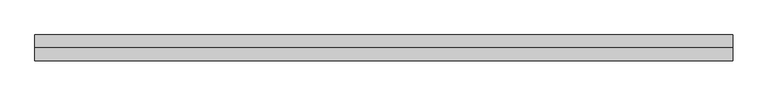
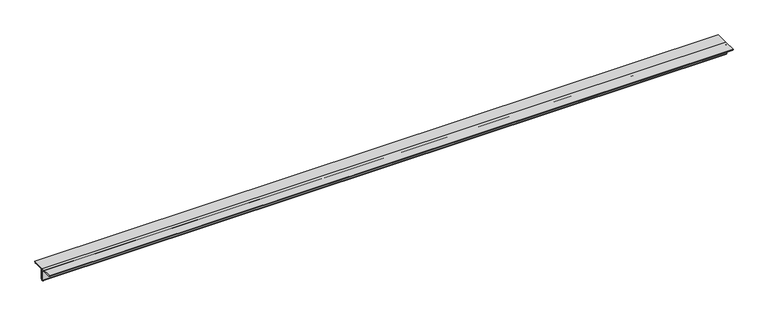
"""IFC4 building model written with IfcOpenShell, lengths in millimetres: member geometry, Steel Framing_2Ls_KS : H_SB_AR_S02_2Ls-100x100x10_VBR1."""

from ifc_helpers import new_model, si_unit, point, frame, frame_2d, origin, place, context, project, spatial, polyline, circle_curve, trimmed, segment, composite_curve, outline, extrude, source, transform, mapped, element, save


def member_a8eb377e(model_context):
    return source(origin(), model_context, "Body", "SweptSolid", [
        extrude(outline(composite_curve([segment(polyline([(0.0, 28.2), (0.0, -71.8)]), True, "CONTINUOUS"), segment(trimmed(circle_curve(frame_2d((0.0, -61.8)), 10.0), [point((0.0, -71.8))], [point((-10.0, -61.8))], False, "CARTESIAN"), True, "CONTINUOUS"), segment(polyline([(-10.0, -61.8), (-10.0, 8.2)]), True, "CONTINUOUS"), segment(trimmed(circle_curve(frame_2d((-20.0, 8.2)), 10.0), [point((-10.0, 8.2))], [point((-20.0, 18.2))], True, "CARTESIAN"), True, "CONTINUOUS"), segment(polyline([(-20.0, 18.2), (-90.0, 18.2)]), True, "CONTINUOUS"), segment(trimmed(circle_curve(frame_2d((-90.0, 28.2)), 10.0), [point((-90.0, 18.2))], [point((-100.0, 28.2))], False, "CARTESIAN"), True, "CONTINUOUS"), segment(polyline([(-100.0, 28.2), (0.0, 28.2)]), True, "CONTINUOUS")], self_intersect=False)), frame((-2765.2972366, 0.0, 0.0), z_axis=(1.0, 0.0, 0.0), x_axis=(0.0, 1.0, 0.0)), (0.0, 0.0, 1.0), 5399.8099488),
        extrude(outline(composite_curve([segment(polyline([(0.0, 28.2), (100.0, 28.2)]), True, "CONTINUOUS"), segment(trimmed(circle_curve(frame_2d((90.0, 28.2)), 10.0), [point((100.0, 28.2))], [point((90.0, 18.2))], False, "CARTESIAN"), True, "CONTINUOUS"), segment(polyline([(90.0, 18.2), (20.0, 18.2)]), True, "CONTINUOUS"), segment(trimmed(circle_curve(frame_2d((20.0, 8.2)), 10.0), [point((20.0, 18.2))], [point((10.0, 8.2))], True, "CARTESIAN"), True, "CONTINUOUS"), segment(polyline([(10.0, 8.2), (10.0, -61.8)]), True, "CONTINUOUS"), segment(trimmed(circle_curve(frame_2d((0.0, -61.8)), 10.0), [point((10.0, -61.8))], [point((0.0, -71.8))], False, "CARTESIAN"), True, "CONTINUOUS"), segment(polyline([(0.0, -71.8), (0.0, 28.2)]), True, "CONTINUOUS")], self_intersect=False)), frame((-2765.2972366, 0.0, 0.0), z_axis=(1.0, 0.0, 0.0), x_axis=(0.0, 1.0, 0.0)), (0.0, 0.0, 1.0), 5399.8099488),
    ])


if __name__ == "__main__":
    model = new_model("IFC4")
    model_context = context("Model", 3, world=origin())
    ifc_project = project(units=[si_unit("LENGTHUNIT", "METRE", prefix="MILLI")], contexts=[model_context])
    site = spatial("IfcSite", under=ifc_project)
    building = spatial("IfcBuilding", under=site)
    placement = place(None, origin())
    member_shape = member_a8eb377e(model_context)
    element("IfcMember", 1, ObjectType="Steel Framing_2Ls_KS : H_SB_AR_S02_2Ls-100x100x10_VBR1", at=placement, inside=building, context=model_context, shape_type="MappedRepresentation", body=[
        mapped(member_shape, transform((0.0, 0.0, 0.0), x_axis=(1.0, 0.0, 0.0), y_axis=(0.0, 1.0, 0.0), z_axis=(0.0, 0.0, 1.0))),
    ])
    save(model, "model.ifc")

# Revit data of these elements
# Type "Steel Framing_2Ls_KS : H_SB_AR_S02_2Ls-100x100x10_VBR1"
#   Type Comments = "MAIN"
#   Type Mark = "VBR1"
#   H_SectionID = "2Ls-100x100x10"
#   Assembly Code = "B10"
#   Legs = "LLBB"
#   H_Ratio for Additional Steel Plate = 0.2
#   W = 0
#   Perimeter = 0.80 m²/m
#   Nominal Weight = 29.80 kgf/m
#   Length [instance default] = 1524 mm
#   Space = 0 mm
#   b = 100 mm
#   d = 100 mm
#   t = 10 mm
#   y = 28.2 mm
#   A = 0.0038 m²
#   Structural Material [instance default] = Steel, 45-345
# Element 1 (IfcMember, "Steel Framing_2Ls_KS : H_SB_AR_S02_2Ls-100x100x10_VBR1")
#   Materials on its faces: "Steel, 45-345"
# Materials
#   "Steel, 45-345": class "Metal", colour RGB 189 187 185, transparency 0, Description = "Steel 345 MPa", Cost = 0
